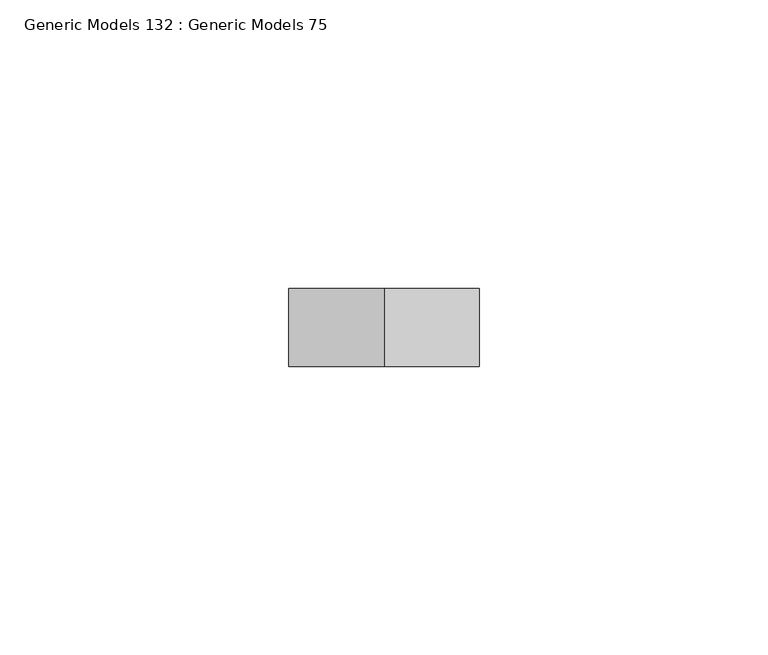
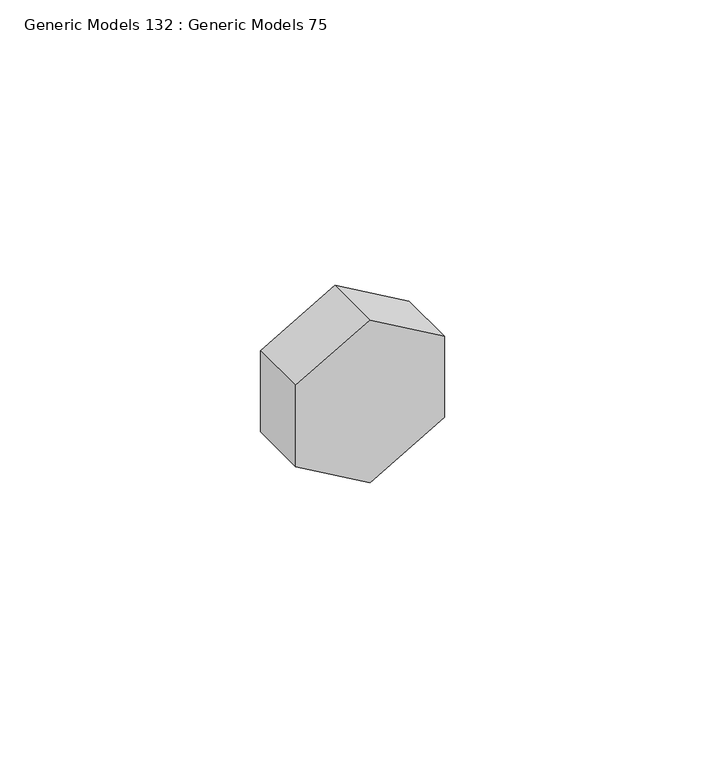
"""IFC4 building model written with IfcOpenShell, lengths in millimetres: proxy geometry, Generic Models 132 : Generic Models 75."""

from ifc_helpers import new_model, si_unit, frame, origin, place, context, project, spatial, polyline, outline, extrude, source, transform, mapped, element, save


def generic_models_132_generic_models_75_c0152725(model_context):
    return source(origin(), model_context, "Body", "SweptSolid", [
        extrude(outline(polyline([(268485.9375, 31991.9073871), (268504.9875, 31991.9073871), (268514.5125, 31975.4096032), (268504.9875, 31958.9118192), (268485.9375, 31958.9118192), (268476.4125, 31975.4096032), (268485.9375, 31991.9073871)])), frame((0.0, 33977.9585924, 0.0), z_axis=(0.0, 1.0, 0.0), x_axis=(0.0, 0.0, 1.0)), (0.0, 0.0, 1.0), 13.49375),
    ])


if __name__ == "__main__":
    model = new_model("IFC4")
    model_context = context("Model", 3, world=origin())
    ifc_project = project(units=[si_unit("LENGTHUNIT", "METRE", prefix="MILLI")], contexts=[model_context])
    site = spatial("IfcSite", under=ifc_project)
    building = spatial("IfcBuilding", under=site)
    placement = place(None, origin())
    generic_models_132_generic_models_75_shape = generic_models_132_generic_models_75_c0152725(model_context)
    element("IfcBuildingElementProxy", 1, Name="Generic Models 132 : Generic Models 75", ObjectType="Generic Models 132 : Generic Models 75", at=placement, inside=building, context=model_context, shape_type="MappedRepresentation", body=[
        mapped(generic_models_132_generic_models_75_shape, transform((0.0, 0.0, 0.0), x_axis=(1.0, 0.0, 0.0), y_axis=(0.0, 1.0, 0.0), z_axis=(0.0, 0.0, 1.0))),
    ])
    save(model, "model.ifc")
